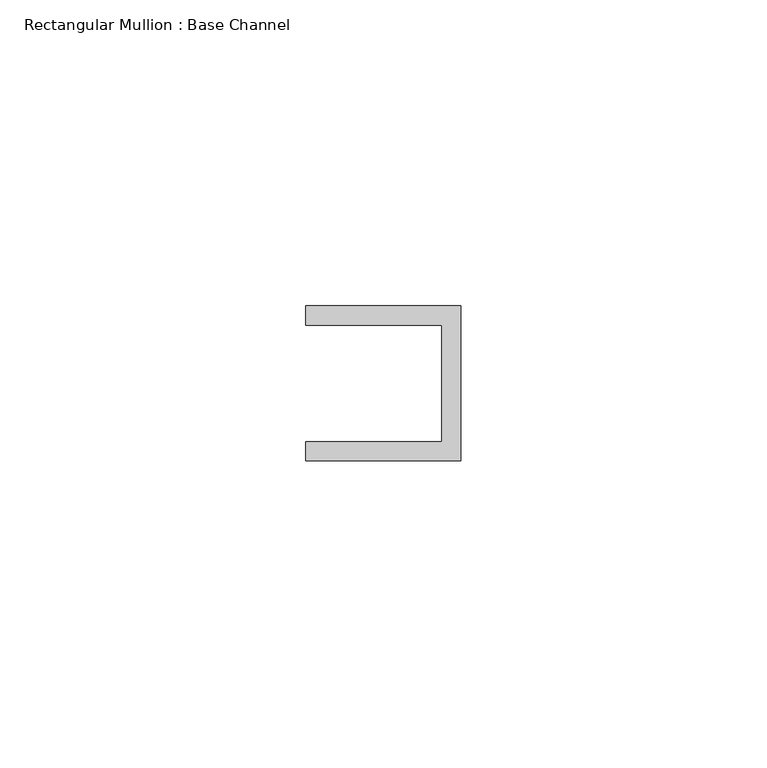
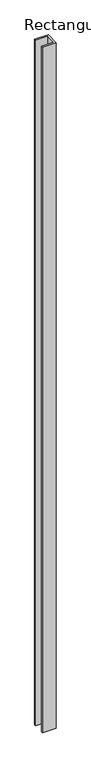
"""IFC4 building model written with IfcOpenShell, lengths in millimetres: member geometry, Rectangular Mullion : Base Channel."""

from ifc_helpers import new_model, si_unit, frame, origin, place, context, project, spatial, polyline, outline, extrude, source, transform, mapped, element, save


def rectangular_mullion_base_channel_9abaf7b8(model_context):
    return source(origin(), model_context, "Body", "SweptSolid", [
        extrude(outline(polyline([(0.0, 12.7), (0.0, -12.7), (-25.4, -12.7), (-25.4, -9.525), (-3.175, -9.525), (-3.175, 9.525), (-25.4, 9.525), (-25.4, 12.7), (0.0, 12.7)])), frame((0.0, 0.0, -1346.2), z_axis=(0.0, 0.0, 1.0), x_axis=(1.0, 0.0, 0.0)), (0.0, 0.0, 1.0), 1346.2),
    ])


if __name__ == "__main__":
    model = new_model("IFC4")
    model_context = context("Model", 3, world=origin())
    ifc_project = project(units=[si_unit("LENGTHUNIT", "METRE", prefix="MILLI")], contexts=[model_context])
    site = spatial("IfcSite", under=ifc_project)
    building = spatial("IfcBuilding", under=site)
    placement = place(None, origin())
    rectangular_mullion_base_channel_shape = rectangular_mullion_base_channel_9abaf7b8(model_context)
    element("IfcMember", 1, ObjectType="Rectangular Mullion : Base Channel", at=placement, inside=building, context=model_context, shape_type="MappedRepresentation", body=[
        mapped(rectangular_mullion_base_channel_shape, transform((0.0, 0.0, 0.0), x_axis=(1.0, 0.0, 0.0), y_axis=(0.0, 1.0, 0.0), z_axis=(0.0, 0.0, 1.0))),
    ])
    save(model, "model.ifc")

# Revit data of these elements
# Type "Rectangular Mullion : Base Channel"
#   built-in parameter 1007322 = 0.0833333 (stored number, unit not read)
#   built-in parameter 1007321 = 0.0416667 (stored number, unit not read)
#   built-in parameter 1007320 = -0.03125 (stored number, unit not read)
# Element 1 (IfcMember, "Rectangular Mullion : Base Channel")
#   Materials on its faces: "ALUM"
# Materials
#   "ALUM": class "Generic", colour RGB 157 157 157, transparency 0, Cost = 0
